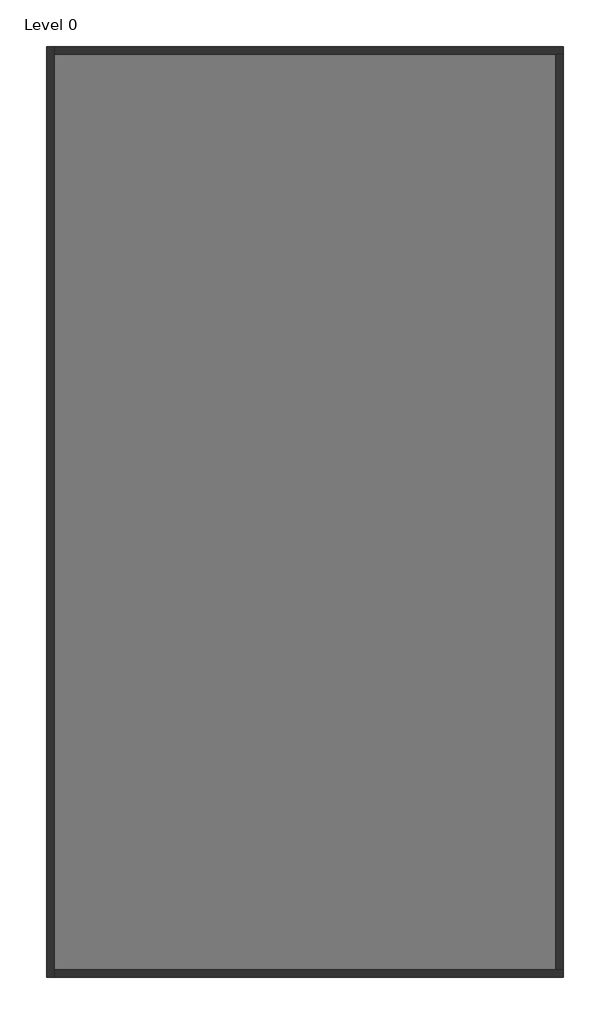
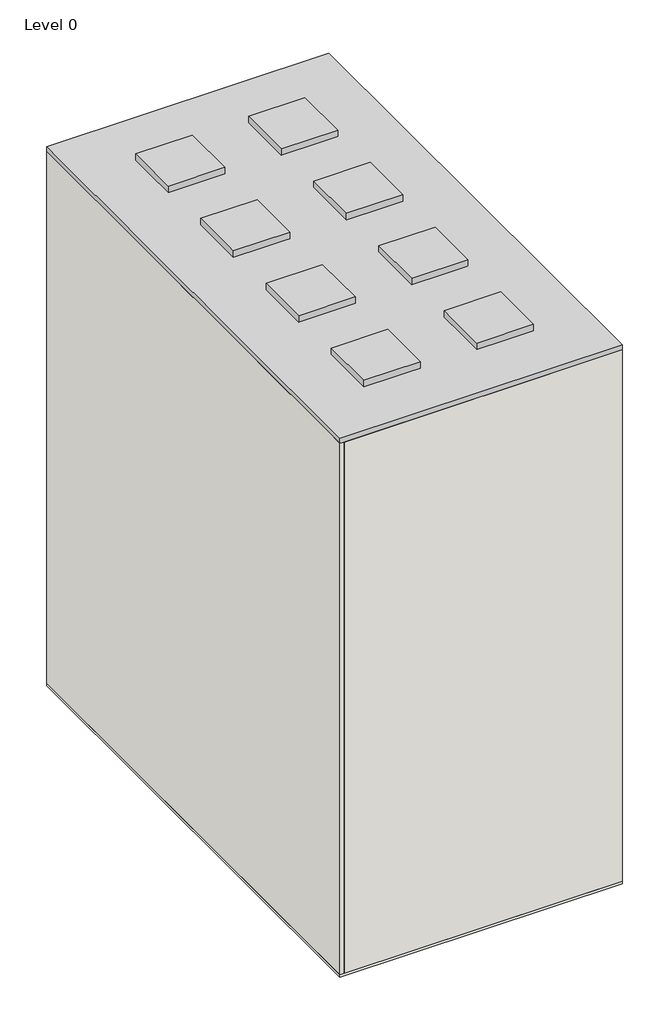
# One storey: 4 walls, 1 proxy, 1 slab.
"""IFC4 building model written with IfcOpenShell, lengths in millimetres."""

from ifc_helpers import new_model, si_unit, frame, origin, origin_with_axes, place, context, project, spatial, polyline, outline, extrude, faceted_brep, element, save

model = new_model("IFC4")

# Units and contexts
model_context = context("Model", 3, world=origin())
ifc_project = project(units=[si_unit("LENGTHUNIT", "METRE", prefix="MILLI")], contexts=[model_context])

# Site, building, storey
site = spatial("IfcSite", under=ifc_project)
building = spatial("IfcBuilding", under=site)
storey = spatial("IfcBuildingStorey", under=building, Name="Level 0", Elevation=100.0)

# Proxy
placement = place(None, origin())
element("IfcBuildingElementProxy", 1, Name="LowUrbanDensityBuilding : LowUrbanDensityBuilding", ObjectType="LowUrbanDensityBuilding : LowUrbanDensityBuilding", at=placement, inside=storey, context=model_context, shape_type="SweptSolid", body=[
    extrude(outline(polyline([(7325.2659446, 3676.2074539), (7325.2659446, -14323.7925461), (-2674.7340554, -14323.7925461), (-2674.7340554, 3676.2074539), (7325.2659446, 3676.2074539)])), origin_with_axes(), (0.0, 0.0, 1.0), 20200.0),
    extrude(outline(polyline([(1325.2659446, 1676.2074539), (1325.2659446, -323.7925461), (-674.7340554, -323.7925461), (-674.7340554, 1676.2074539), (1325.2659446, 1676.2074539)])), frame((0.0, 0.0, 20200.0), z_axis=(0.0, 0.0, 1.0), x_axis=(1.0, 0.0, 0.0)), (0.0, 0.0, 1.0), 245.0),
    extrude(outline(polyline([(5325.2659446, 1676.2074539), (5325.2659446, -323.7925461), (3325.2659446, -323.7925461), (3325.2659446, 1676.2074539), (5325.2659446, 1676.2074539)])), frame((0.0, 0.0, 20200.0), z_axis=(0.0, 0.0, 1.0), x_axis=(1.0, 0.0, 0.0)), (0.0, 0.0, 1.0), 245.0),
    extrude(outline(polyline([(1325.2659446, -2323.7925461), (1325.2659446, -4323.7925461), (-674.7340554, -4323.7925461), (-674.7340554, -2323.7925461), (1325.2659446, -2323.7925461)])), frame((0.0, 0.0, 20200.0), z_axis=(0.0, 0.0, 1.0), x_axis=(1.0, 0.0, 0.0)), (0.0, 0.0, 1.0), 245.0),
    extrude(outline(polyline([(5325.2659446, -2323.7925461), (5325.2659446, -4323.7925461), (3325.2659446, -4323.7925461), (3325.2659446, -2323.7925461), (5325.2659446, -2323.7925461)])), frame((0.0, 0.0, 20200.0), z_axis=(0.0, 0.0, 1.0), x_axis=(1.0, 0.0, 0.0)), (0.0, 0.0, 1.0), 245.0),
    extrude(outline(polyline([(1325.2659446, -6323.7925461), (1325.2659446, -8323.7925461), (-674.7340554, -8323.7925461), (-674.7340554, -6323.7925461), (1325.2659446, -6323.7925461)])), frame((0.0, 0.0, 20200.0), z_axis=(0.0, 0.0, 1.0), x_axis=(1.0, 0.0, 0.0)), (0.0, 0.0, 1.0), 245.0),
    extrude(outline(polyline([(5325.2659446, -6323.7925461), (5325.2659446, -8323.7925461), (3325.2659446, -8323.7925461), (3325.2659446, -6323.7925461), (5325.2659446, -6323.7925461)])), frame((0.0, 0.0, 20200.0), z_axis=(0.0, 0.0, 1.0), x_axis=(1.0, 0.0, 0.0)), (0.0, 0.0, 1.0), 245.0),
    extrude(outline(polyline([(1325.2659446, -10323.7925461), (1325.2659446, -12323.7925461), (-674.7340554, -12323.7925461), (-674.7340554, -10323.7925461), (1325.2659446, -10323.7925461)])), frame((0.0, 0.0, 20200.0), z_axis=(0.0, 0.0, 1.0), x_axis=(1.0, 0.0, 0.0)), (0.0, 0.0, 1.0), 245.0),
    extrude(outline(polyline([(5325.2659446, -10323.7925461), (5325.2659446, -12323.7925461), (3325.2659446, -12323.7925461), (3325.2659446, -10323.7925461), (5325.2659446, -10323.7925461)])), frame((0.0, 0.0, 20200.0), z_axis=(0.0, 0.0, 1.0), x_axis=(1.0, 0.0, 0.0)), (0.0, 0.0, 1.0), 245.0),
])

# Slab
element("IfcSlab", 2, ObjectType="Floor-Concrete_100Con", at=placement, inside=storey, context=model_context, shape_type="SweptSolid", body=[
    extrude(outline(polyline([(7325.2659446, 3676.2074539), (7325.2659446, -14323.7925461), (-2674.7340554, -14323.7925461), (-2674.7340554, 3676.2074539), (7325.2659446, 3676.2074539)])), origin_with_axes(), (0.0, 0.0, 1.0), 100.0),
])

# Walls
element("IfcWall", 3, ObjectType="Wall-Ext_25Rdr-100Blk-19P", at=placement, inside=storey, context=model_context, shape_type="Brep", body=[
    faceted_brep([(-2674.7340554, 3676.2074539, 100.0), (-2674.7340554, -14323.7925461, 100.0), (-2674.7340554, -14323.7925461, 20000.0), (-2674.7340554, 3676.2074539, 20000.0), (-2530.4340554, 3676.2074539, 100.0), (-2530.4340554, 3676.2074539, 20000.0), (-2530.4340554, 3531.9074539, 20000.0), (-2530.4340554, -14179.4925461, 20000.0), (-2530.4340554, -14323.7925461, 20000.0), (-2530.4340554, -14323.7925461, 100.0), (-2530.4340554, -14179.4925461, 100.0), (-2530.4340554, 3531.9074539, 100.0)], [[[0, 1, 2, 3]], [[4, 5, 6, 7, 8, 9, 10, 11]], [[1, 0, 4, 11, 10, 9]], [[3, 2, 8, 7, 6, 5]], [[2, 1, 9, 8]], [[0, 3, 5, 4]]]),
])
element("IfcWall", 4, ObjectType="Wall-Ext_25Rdr-100Blk-19P", at=placement, inside=storey, context=model_context, shape_type="Brep", body=[
    faceted_brep([(-2530.4340554, -14323.7925461, 100.0), (7325.2659446, -14323.7925461, 100.0), (7325.2659446, -14323.7925461, 20000.0), (-2530.4340554, -14323.7925461, 20000.0), (-2530.4340554, -14179.4925461, 100.0), (-2530.4340554, -14179.4925461, 20000.0), (7180.9659446, -14179.4925461, 20000.0), (7325.2659446, -14179.4925461, 20000.0), (7325.2659446, -14179.4925461, 100.0), (7180.9659446, -14179.4925461, 100.0)], [[[0, 1, 2, 3]], [[4, 5, 6, 7, 8, 9]], [[1, 0, 4, 9, 8]], [[3, 2, 7, 6, 5]], [[0, 3, 5, 4]], [[2, 1, 8, 7]]]),
])
element("IfcWall", 5, ObjectType="Wall-Ext_25Rdr-100Blk-19P", at=placement, inside=storey, context=model_context, shape_type="Brep", body=[
    faceted_brep([(7325.2659446, 3676.2074539, 100.0), (-2530.4340554, 3676.2074539, 100.0), (-2530.4340554, 3676.2074539, 20000.0), (7325.2659446, 3676.2074539, 20000.0), (7325.2659446, 3531.9074539, 100.0), (7325.2659446, 3531.9074539, 20000.0), (7180.9659446, 3531.9074539, 20000.0), (-2530.4340554, 3531.9074539, 20000.0), (-2530.4340554, 3531.9074539, 100.0), (7180.9659446, 3531.9074539, 100.0)], [[[0, 1, 2, 3]], [[4, 5, 6, 7, 8, 9]], [[1, 0, 4, 9, 8]], [[3, 2, 7, 6, 5]], [[2, 1, 8, 7]], [[0, 3, 5, 4]]]),
])
element("IfcWall", 6, ObjectType="Wall-Ext_25Rdr-100Blk-19P", at=placement, inside=storey, context=model_context, shape_type="SweptSolid", body=[
    extrude(outline(polyline([(7325.2659446, 3531.9074539), (7325.2659446, -14179.4925461), (7180.9659446, -14179.4925461), (7180.9659446, 3531.9074539), (7325.2659446, 3531.9074539)])), frame((0.0, 0.0, 100.0), z_axis=(0.0, 0.0, 1.0), x_axis=(1.0, 0.0, 0.0)), (0.0, 0.0, 1.0), 19900.0),
])

save(model, "model.ifc")

# Revit data of these elements
# Project information
#   Project Issue Date = "Issue Date"
#   Project Status = "Project Status"
#   Client Name = "Owner"
#   Project Address = "Enter address here"
#   Project Name = "Project Name"
#   Project Number = "Project Number"
# Type "Floor-Concrete_100Con"
#   Keynote = "E60/130"
#   Function = 0
#   Layers, outside or top first: 100 mm "Concrete" (function 1)
# Type "Wall-Ext_25Rdr-100Blk-19P"
#   Keynote = "F10"
#   Layers, outside or top first: 25.3 mm "Render, Beige, Smooth" (function 5); 100 mm "Concrete Masonry Units _Low Density" (function 1); 19 mm "Plaster" (function 5)
# Element 1 (IfcBuildingElementProxy, "LowUrbanDensityBuilding : LowUrbanDensityBuilding")
#   Phase Created = New Construction
#   Materials on its faces: "Default Form"
# Element 2 (IfcSlab, "Floor-Concrete_100Con")
#   Height Offset From Level = 0 mm
#   Phase Created = New Construction
#   Materials on its faces: "Concrete"
# Element 3 (IfcWall, "Wall-Ext_25Rdr-100Blk-19P")
#   Top Offset = 0 mm
#   Base Offset = 0 mm
#   wall height = 19900 mm
#   Phase Created = New Construction
#   Base Constraint = Level 0
#   Top Constraint = Level 5
#   Materials on its faces: "Render, Beige, Smooth", "Default Wall", "Plaster"
# Elements 4, 5, 6 (IfcWall, "Wall-Ext_25Rdr-100Blk-19P")
#   Top Offset = 0 mm
#   Base Offset = 0 mm
#   wall height = 19900 mm
#   Phase Created = New Construction
#   Base Constraint = Level 0
#   Top Constraint = Level 5
#   Materials on its faces: "Default Wall", "Render, Beige, Smooth", "Plaster"
# Materials
#   "Concrete": class "Concrete", colour RGB 120 120 120, transparency 0, Description = "Portland Cement Concrete", Cost = 0
#   "Render, Beige, Smooth": class "Generic", colour RGB 213 198 180, transparency 0, Description = "physical material", Cost = 0
#   "Concrete Masonry Units _Low Density": class "Masonry", colour RGB 181 181 181, transparency 0, Description = "Concrete masonry units", Cost = 0
#   "Plaster": class "Generic", colour RGB 249 249 249, transparency 0, Description = "Plaster", Cost = 0
#   "Default Form": class "Generic", colour RGB 185 189 196, transparency 0.5, Cost = 0
#   "Default Wall": class "Miscellaneous", colour RGB 128 128 128, transparency 0, Comments = "Rendering appearance not upgraded Rendering appearance not upgraded ", Cost = 0
